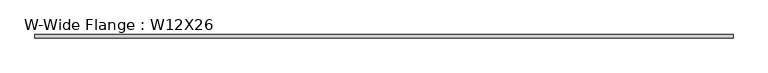
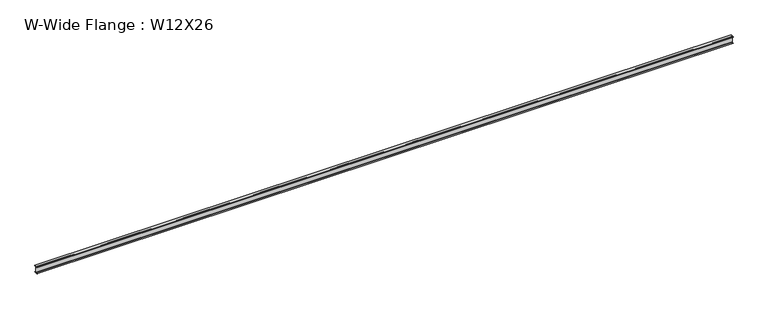
"""IFC4 building model written with IfcOpenShell, lengths in millimetres: beam geometry, W-Wide Flange : W12X26."""

from ifc_helpers import new_model, si_unit, point, frame, frame_2d, origin, place, context, project, spatial, polyline, circle_curve, trimmed, segment, composite_curve, outline, extrude, source, transform, mapped, element, save


def w_wide_flange_w12x26_43b49b8e(model_context):
    return source(origin(), model_context, "Body", "SweptSolid", [
        extrude(outline(composite_curve([segment(polyline([(82.4011719, -145.5539063), (82.4011719, -155.178125), (-82.4011719, -155.178125), (-82.4011719, -145.5539063), (-20.2902344, -145.5539063)]), True, "CONTINUOUS"), segment(trimmed(circle_curve(frame_2d((-20.2902344, -128.190625)), 17.3632812), [point((-20.2902344, -145.5539063))], [point((-2.9269531, -128.190625))], True, "CARTESIAN"), True, "CONTINUOUS"), segment(polyline([(-2.9269531, -128.190625), (-2.9269531, 128.190625)]), True, "CONTINUOUS"), segment(trimmed(circle_curve(frame_2d((-20.2902344, 128.190625)), 17.3632812), [point((-2.9269531, 128.190625))], [point((-20.2902344, 145.5539062))], True, "CARTESIAN"), True, "CONTINUOUS"), segment(polyline([(-20.2902344, 145.5539062), (-82.4011719, 145.5539062), (-82.4011719, 155.178125), (82.4011719, 155.178125), (82.4011719, 145.5539062), (20.2902344, 145.5539062)]), True, "CONTINUOUS"), segment(trimmed(circle_curve(frame_2d((20.2902344, 128.190625)), 17.3632812), [point((20.2902344, 145.5539062))], [point((2.9269531, 128.190625))], True, "CARTESIAN"), True, "CONTINUOUS"), segment(polyline([(2.9269531, 128.190625), (2.9269531, -128.190625)]), True, "CONTINUOUS"), segment(trimmed(circle_curve(frame_2d((20.2902344, -128.190625)), 17.3632812), [point((2.9269531, -128.190625))], [point((20.2902344, -145.5539063))], True, "CARTESIAN"), True, "CONTINUOUS"), segment(polyline([(20.2902344, -145.5539063), (82.4011719, -145.5539063)]), True, "CONTINUOUS")], self_intersect=False)), frame((-16154.4, 0.0, 0.0), z_axis=(1.0, 0.0, 0.0), x_axis=(0.0, 1.0, 0.0)), (0.0, 0.0, 1.0), 32308.8),
    ])


if __name__ == "__main__":
    model = new_model("IFC4")
    model_context = context("Model", 3, world=origin())
    ifc_project = project(units=[si_unit("LENGTHUNIT", "METRE", prefix="MILLI")], contexts=[model_context])
    site = spatial("IfcSite", under=ifc_project)
    building = spatial("IfcBuilding", under=site)
    placement = place(None, origin())
    w_wide_flange_w12x26_shape = w_wide_flange_w12x26_43b49b8e(model_context)
    element("IfcBeam", 1, ObjectType="W-Wide Flange : W12X26", at=placement, inside=building, context=model_context, shape_type="MappedRepresentation", body=[
        mapped(w_wide_flange_w12x26_shape, transform((0.0, 0.0, 0.0), x_axis=(1.0, 0.0, 0.0), y_axis=(0.0, 1.0, 0.0), z_axis=(0.0, 0.0, 1.0))),
    ])
    save(model, "model.ifc")

# Revit data of these elements
# Type "W-Wide Flange : W12X26"
#   Assembly Code = "B10"
#   W = 26
#   Length [instance default] = 5' - 0"
#   bf = 0' - 6 125/256"
#   d = 1' - 0 7/32"
#   k = 0' - 1 1/16"
#   k2 = 0' - 0 175/256"
#   tf = 0' - 0 97/256"
#   tw = 0' - 0 59/256"
#   A = 0.053125 SF
#   Structural Material [instance default] = none
